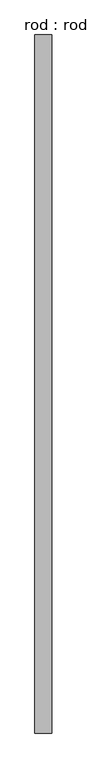
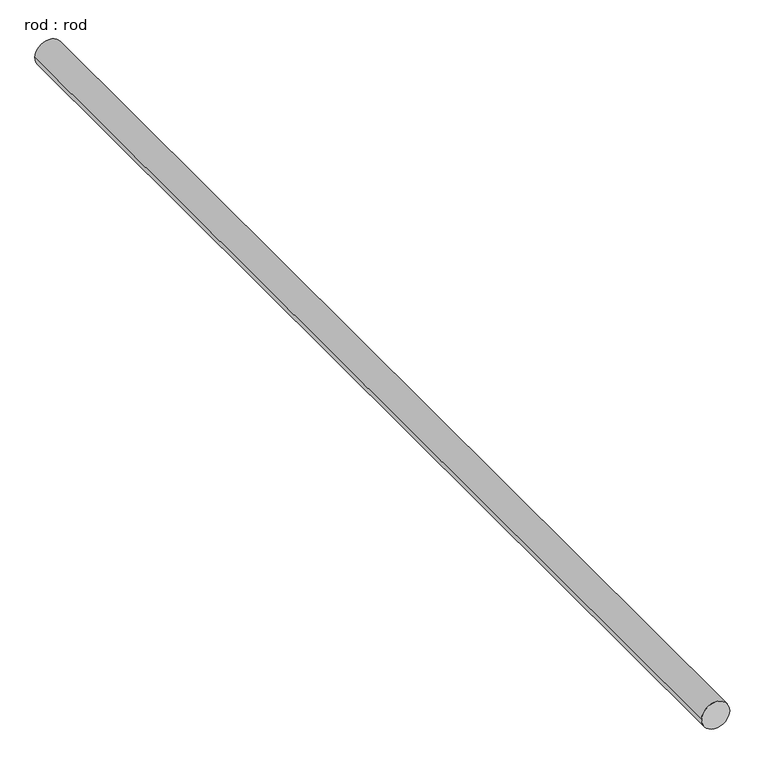
"""IFC4 building model written with IfcOpenShell, lengths in millimetres: proxy geometry, rod : rod."""

from ifc_helpers import new_model, si_unit, point, frame, frame_2d, origin, place, context, project, spatial, circle_curve, trimmed, segment, composite_curve, outline, extrude, source, transform, mapped, element, save


def rod_rod_ca877957(model_context):
    return source(origin(), model_context, "Body", "SweptSolid", [
        extrude(outline(composite_curve([segment(trimmed(circle_curve(frame_2d((0.0108462, 0.0)), 200.0), [point((0.0108462, 200.0))], [point((0.0108462, -200.0))], False, "CARTESIAN"), True, "CONTINUOUS"), segment(trimmed(circle_curve(frame_2d((0.0108462, 0.0)), 200.0), [point((0.0108462, -200.0))], [point((0.0108462, 200.0))], False, "CARTESIAN"), True, "CONTINUOUS")], self_intersect=False)), frame((0.0, -4130.4856704, 0.0), z_axis=(0.0, 1.0, 0.0), x_axis=(0.0, 0.0, 1.0)), (0.0, 0.0, 1.0), 16446.4285714),
    ])


if __name__ == "__main__":
    model = new_model("IFC4")
    model_context = context("Model", 3, world=origin())
    ifc_project = project(units=[si_unit("LENGTHUNIT", "METRE", prefix="MILLI")], contexts=[model_context])
    site = spatial("IfcSite", under=ifc_project)
    building = spatial("IfcBuilding", under=site)
    placement = place(None, origin())
    rod_rod_shape = rod_rod_ca877957(model_context)
    element("IfcBuildingElementProxy", 1, Name="rod : rod", ObjectType="rod : rod", at=placement, inside=building, context=model_context, shape_type="MappedRepresentation", body=[
        mapped(rod_rod_shape, transform((0.0, 0.0, 0.0), x_axis=(1.0, 0.0, 0.0), y_axis=(0.0, 1.0, 0.0), z_axis=(0.0, 0.0, 1.0))),
    ])
    save(model, "model.ifc")

# Revit data of these elements
# Type "rod : rod"
#   Default Elevation = 0
